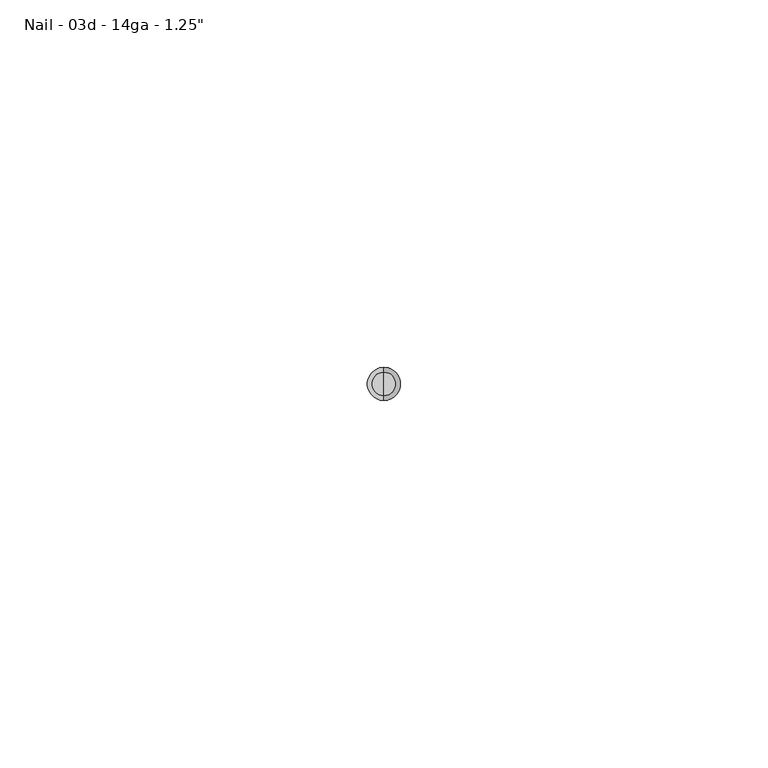
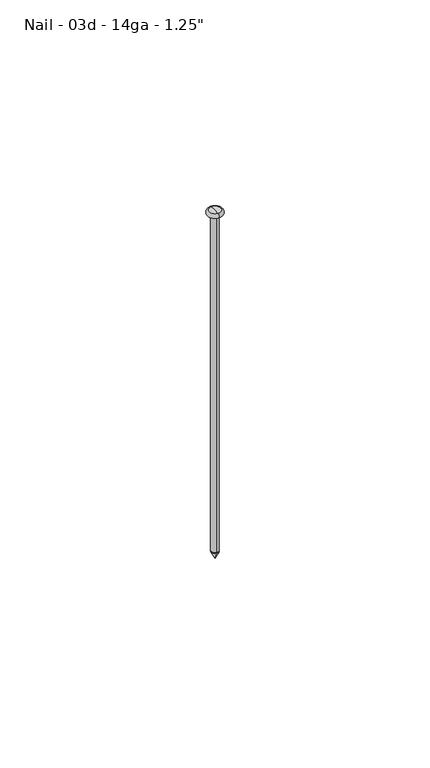
"""IFC4 building model written with IfcOpenShell, lengths in millimetres: fastener geometry."""

from ifc_helpers import new_model, si_unit, point, frame, origin, origin_2d, place, context, project, spatial, polyline, circle_curve, ellipse_curve, trimmed, segment, composite_curve, outline, extrude, source, transform, mapped, element, save
from ifc_brep_helpers import plane_surface, revolved_surface, advanced_brep


def fastener_acbd573c(model_context):
    return source(origin(), model_context, "Body", "SolidModel", [
        advanced_brep(
        [(0.0, -1.0541, -101.6), (0.0, 1.0541, -101.6), (0.0, 0.0, -101.6), (0.0, 0.0, -103.7082)],
        [
            (0, 1, circle_curve(frame((0.0, 0.0, -101.6), z_axis=(0.0, 0.0, 1.0), x_axis=(0.0, 1.0, 0.0)), 1.0541)),
            (1, 2),
            (2, 0),
            (1, 0, circle_curve(frame((0.0, 0.0, -101.6), z_axis=(0.0, 0.0, 1.0), x_axis=(0.0, 1.0, 0.0)), 1.0541)),
            (3, 1),
            (0, 3),
        ],
        [
            plane_surface(frame((0.0, 0.0, -101.6), z_axis=(0.0, 0.0, 1.0), x_axis=(0.0, 1.0, 0.0))),
            revolved_surface(polyline([(0.0, 1.0541, -101.6), (0.0, 0.0, -103.7082)]), (0.0, 0.0, -103.0840259), (0.0, 0.0, -1.0)),
        ],
        [
            (0, [[1, 2, 3]]),
            (0, [[4, -3, -2]]),
            (1, [[5, -1, 6]]),
            (1, [[-6, -4, -5]]),
        ],
    ),
        advanced_brep(
        [(0.0, 2.1082, 0.0), (0.0, -2.1082, 0.0), (0.0, 0.0, 0.0), (0.0, 0.0, 1.0541), (0.0, -1.5875, 1.0541), (0.0, 1.5875, 1.0541)],
        [
            (0, 1, circle_curve(frame((0.0, 0.0, 0.0), z_axis=(0.0, 0.0, -1.0), x_axis=(0.0, -1.0, 0.0)), 2.1082)),
            (1, 2),
            (2, 0),
            (1, 0, circle_curve(frame((0.0, 0.0, 0.0), z_axis=(0.0, 0.0, -1.0), x_axis=(0.0, -1.0, 0.0)), 2.1082)),
            (3, 4),
            (4, 5, circle_curve(frame((0.0, 0.0, 1.0541), z_axis=(0.0, 0.0, 1.0), x_axis=(0.0, -1.0, 0.0)), 1.5875)),
            (5, 3),
            (5, 4, circle_curve(frame((0.0, 0.0, 1.0541), z_axis=(0.0, 0.0, 1.0), x_axis=(0.0, -1.0, 0.0)), 1.5875)),
            (4, 1, circle_curve(frame((0.0, -1.5875, 0.3984434), z_axis=(1.0, 0.0, 0.0), x_axis=(0.0, -1.0, 0.0)), 0.6556566)),
            (0, 5, circle_curve(frame((0.0, 1.5875, 0.3984434), z_axis=(1.0, 0.0, 0.0), x_axis=(0.0, 1.0, 0.0)), 0.6556566)),
        ],
        [
            plane_surface(frame((0.0, 0.0, 0.0), z_axis=(0.0, 0.0, -1.0), x_axis=(0.0, -1.0, 0.0))),
            plane_surface(frame((0.0, 0.0, 1.0541), z_axis=(0.0, 0.0, 1.0), x_axis=(0.0, -1.0, 0.0))),
            revolved_surface(trimmed(ellipse_curve(frame((0.0, -1.5875, 0.3984434), z_axis=(-1.0, 0.0, 0.0), x_axis=(0.0, -1.0, 0.0)), 0.6556566, 0.6556566), [point((0.0, -2.1082, 0.0))], [point((0.0, -1.5875, 1.0541))], True, "CARTESIAN"), (0.0, 0.0, 1.4840259), (0.0, 0.0, 1.0)),
        ],
        [
            (0, [[1, 2, 3]]),
            (0, [[4, -3, -2]]),
            (1, [[5, 6, 7]]),
            (1, [[-7, 8, -5]]),
            (2, [[-6, 9, -1, 10]]),
            (2, [[-8, -10, -4, -9]]),
        ],
    ),
        extrude(outline(composite_curve([segment(trimmed(circle_curve(origin_2d(), 1.0541), [point((0.0, -1.0541))], [point((0.0, 1.0541))], False, "CARTESIAN"), True, "CONTINUOUS"), segment(trimmed(circle_curve(origin_2d(), 1.0541), [point((0.0, 1.0541))], [point((0.0, -1.0541))], False, "CARTESIAN"), True, "CONTINUOUS")], self_intersect=False)), frame((0.0, 0.0, -101.6), z_axis=(0.0, 0.0, 1.0), x_axis=(1.0, 0.0, 0.0)), (0.0, 0.0, 1.0), 101.6),
    ])


if __name__ == "__main__":
    model = new_model("IFC4")
    model_context = context("Model", 3, world=origin())
    ifc_project = project(units=[si_unit("LENGTHUNIT", "METRE", prefix="MILLI")], contexts=[model_context])
    site = spatial("IfcSite", under=ifc_project)
    building = spatial("IfcBuilding", under=site)
    placement = place(None, origin())
    fastener_shape = fastener_acbd573c(model_context)
    element("IfcFastener", 1, ObjectType="060523 - W_P_C - Fastenings - Generic : Nail - 03d - 14ga - 1.25\"", at=placement, inside=building, context=model_context, shape_type="MappedRepresentation", body=[
        mapped(fastener_shape, transform((0.0, 0.0, 0.0), x_axis=(1.0, 0.0, 0.0), y_axis=(0.0, 1.0, 0.0), z_axis=(0.0, 0.0, 1.0))),
    ])
    save(model, "model.ifc")

# Revit data of these elements
# Type "060523 - W_P_C - Fastenings - Generic : Nail - 03d - 14ga - 1.25\""
#   Washer_Thickness = 0' - 0.00333"
#   Washer Radius = 0' - 0.0515"
#   Washer Offset - Head = 0' - 0"
#   Washer Offset = 0' - 0"
#   Thickness_of_Substrate [instance default] = 0' - 1"
#   Side = 0' - 0 37/64"
#   Radius = 0' - 0.0415"
#   Length [instance default] = 0' - 1 1/4"
#   Head Size = 0' - 1"
#   Head Radius = 0' - 0 1/2"
#   Head Height = 0' - 0.01"
#   Double Diameter = 0' - 0.166"
#   Diameter = 0' - 0.083"
#   Default Elevation = 4' - 0"
#   Washer_Nut_Visibility = no
#   Washer_Head_Visibility = no
#   Round_Head_Visibility = yes
#   Point Visibility = yes
#   Nut_Visibility = no
#   Hex_Head_Visiblilty = no
#   Washer Material = none
#   Bolt Material (Size) = AT SILL - FASTENER AT 24" O.C.
# Element 1 (IfcFastener, "060523 - W_P_C - Fastenings - Generic : Nail - 03d - 14ga - 1.25\"")
#   Length = 0' - 4"
#   Materials on its faces: "AT SILL - FASTENER AT 24\" O.C."
# Materials
#   "AT SILL - FASTENER AT 24\" O.C.": class "Generic", colour RGB 120 120 120, transparency 0, Cost = 0
